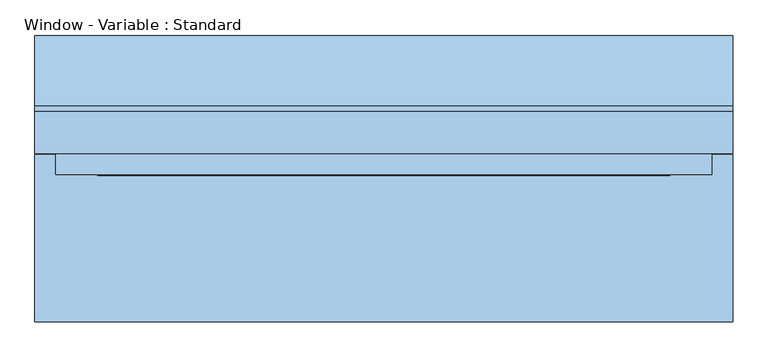
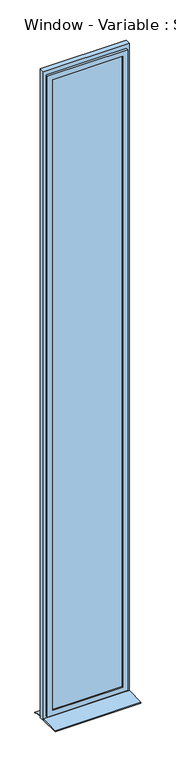
"""IFC4 building model written with IfcOpenShell, lengths in millimetres: window geometry, Window - Variable : Standard."""

import ifcopenshell
import ifcopenshell.guid

model = None  # the IFC model being written
_history = None  # IfcOwnerHistory: only IFC2X3 demands one
_inside = {}  # id of a spatial element -> (the spatial element, [elements in it])
_under = {}  # id of a project, library or spatial element -> (it, [spatial elements below it])
_declared = {}  # id of a project -> (the project, [libraries it declares])
_typed = {}  # id of a type object -> (the type object, [elements of that type])
_made_of = {}  # id of a material, layer set ... -> (it, [elements and type objects made of it])


def new_model(schema):
    """Start an empty IFC model of exactly this schema.

    Asked for "IFC4X3", IfcOpenShell would pick the latest addendum, in which some entities
    have other attributes; the version numbers below select the first issue.
    IFC2X3 requires an IfcOwnerHistory on every rooted entity: one is made here for all.
    """
    global model, _history
    if schema == "IFC4X3":
        model = ifcopenshell.file(schema_version=(4, 3, 0, 0))
    else:
        model = ifcopenshell.file(schema=schema)
    _inside.clear()
    _under.clear()
    _declared.clear()
    _typed.clear()
    _made_of.clear()
    _history = None
    if model.schema == "IFC2X3":
        org = make("IfcOrganization", Name="unknown")
        user = make(
            "IfcPersonAndOrganization",
            ThePerson=make("IfcPerson", FamilyName="unknown"),
            TheOrganization=org,
        )
        app = make(
            "IfcApplication",
            ApplicationDeveloper=org,
            Version="unknown",
            ApplicationFullName="unknown",
            ApplicationIdentifier="unknown",
        )
        _history = make(
            "IfcOwnerHistory",
            OwningUser=user,
            OwningApplication=app,
            ChangeAction="ADDED",
            CreationDate=0,
        )
    return model


def make(cls, **values):
    """One entity of the class cls with the attributes given. An attribute that is None is left unset."""
    return model.create_entity(
        cls, **{name: value for name, value in values.items() if value is not None}
    )


def rooted(cls, **values):
    """An entity with a GlobalId (a new one), such as an element, a storey or a relation."""
    return make(cls, GlobalId=ifcopenshell.guid.new(), OwnerHistory=_history, **values)


def si_unit(unit_type, name, prefix=None):
    """IfcSIUnit, for example si_unit("LENGTHUNIT", "METRE", prefix="MILLI")."""
    return make("IfcSIUnit", UnitType=unit_type, Prefix=prefix, Name=name)


def assignment(units):
    """IfcUnitAssignment: the units of a project."""
    return None if units is None else make("IfcUnitAssignment", Units=units)


def point(xyz):
    """IfcCartesianPoint."""
    return None if xyz is None else make("IfcCartesianPoint", Coordinates=xyz)


def direction(xyz):
    """IfcDirection."""
    return None if xyz is None else make("IfcDirection", DirectionRatios=xyz)


def frame(location, z_axis=None, x_axis=None):
    """IfcAxis2Placement3D, a coordinate frame: its origin and axes. An axis left out is left unset."""
    return make(
        "IfcAxis2Placement3D",
        Location=point(location),
        Axis=direction(z_axis),
        RefDirection=direction(x_axis),
    )


def origin():
    """The frame at (0, 0, 0) with its axes left unset."""
    return frame((0.0, 0.0, 0.0))


def place(relative_to, where):
    """IfcLocalPlacement: puts the frame where relative to a parent placement (None: the world)."""
    return make(
        "IfcLocalPlacement", PlacementRelTo=relative_to, RelativePlacement=where
    )


def context(
    kind, dimensions, precision=None, world=None, true_north=None, identifier=None
):
    """IfcGeometricRepresentationContext, for example the 3D "Model" context."""
    return make(
        "IfcGeometricRepresentationContext",
        ContextIdentifier=identifier,
        ContextType=kind,
        CoordinateSpaceDimension=dimensions,
        Precision=precision,
        WorldCoordinateSystem=world,
        TrueNorth=true_north,
    )


def project(units=None, contexts=None):
    """IfcProject with its units and contexts."""
    return rooted(
        "IfcProject",
        Name="project",
        RepresentationContexts=contexts,
        UnitsInContext=assignment(units),
    )


def spatial(cls, under=None, at=None, **own):
    """A site, building, storey or space (cls), placed at a placement, below another one or the project."""
    s = rooted(cls, ObjectPlacement=at, **own)
    if under is not None:
        _under.setdefault(under.id(), (under, []))[1].append(s)
    return s


def polyline(points):
    """IfcPolyline through the points."""
    return make("IfcPolyline", Points=[point(p) for p in points])


def outline(outer, holes=None, kind="AREA"):
    """IfcArbitraryClosedProfileDef: a profile drawn as a closed curve; with holes, ...WithVoids."""
    if holes is None:
        return make("IfcArbitraryClosedProfileDef", ProfileType=kind, OuterCurve=outer)
    return make(
        "IfcArbitraryProfileDefWithVoids",
        ProfileType=kind,
        OuterCurve=outer,
        InnerCurves=holes,
    )


def extrude(swept, where, along, depth):
    """IfcExtrudedAreaSolid: the profile swept, set in the frame where, extruded along a direction by depth."""
    return make(
        "IfcExtrudedAreaSolid",
        SweptArea=swept,
        Position=where,
        ExtrudedDirection=direction(along),
        Depth=depth,
    )


def faces_of(points, faces, orient=None, outer=None):
    """IfcFace entities. A face is a list of loops; a loop is a list of indices into points, from 0.

    orient and outer hold one flag for each loop. By default every Orientation is true, the
    first loop of a face is its IfcFaceOuterBound and the others are IfcFaceBound.
    """
    made = []
    for i, loops in enumerate(faces):
        bounds = []
        for j, loop in enumerate(loops):
            is_outer = j == 0 if outer is None else outer[i][j]
            bounds.append(
                make(
                    "IfcFaceOuterBound" if is_outer else "IfcFaceBound",
                    Bound=make("IfcPolyLoop", Polygon=[points[k] for k in loop]),
                    Orientation=True if orient is None else orient[i][j],
                )
            )
        made.append(make("IfcFace", Bounds=bounds))
    return made


def faceted_brep(points, faces, orient=None, outer=None, voids=None):
    """IfcFacetedBrep: a solid bounded by flat faces; with voids (closed shells), ...WithVoids."""
    shared = [point(p) for p in points]
    hull = make("IfcClosedShell", CfsFaces=faces_of(shared, faces, orient, outer))
    if voids is None:
        return make("IfcFacetedBrep", Outer=hull)
    return make(
        "IfcFacetedBrepWithVoids",
        Outer=hull,
        Voids=[
            make(cls, CfsFaces=faces_of(shared, fs, o, b)) for cls, fs, o, b in voids
        ],
    )


def shape(context_of_items, identifier, shape_type, items):
    """IfcShapeRepresentation: the items that make up one representation, for example the "Body"."""
    return make(
        "IfcShapeRepresentation",
        ContextOfItems=context_of_items,
        RepresentationIdentifier=identifier,
        RepresentationType=shape_type,
        Items=items,
    )


def source(mapping_origin, context_of_items, identifier, shape_type, items):
    """IfcRepresentationMap: a shape defined once, which mapped items show again and again."""
    return make(
        "IfcRepresentationMap",
        MappingOrigin=mapping_origin,
        MappedRepresentation=shape(context_of_items, identifier, shape_type, items),
    )


def transform(
    local_origin,
    x_axis=None,
    y_axis=None,
    z_axis=None,
    scale=None,
    scale2=None,
    scale3=None,
    uniform=True,
):
    """IfcCartesianTransformationOperator3D, or its non-uniform kind. x_axis, y_axis, z_axis: its Axis1, 2, 3."""
    if uniform:
        return make(
            "IfcCartesianTransformationOperator3D",
            Axis1=direction(x_axis),
            Axis2=direction(y_axis),
            LocalOrigin=point(local_origin),
            Scale=scale,
            Axis3=direction(z_axis),
        )
    return make(
        "IfcCartesianTransformationOperator3DnonUniform",
        Axis1=direction(x_axis),
        Axis2=direction(y_axis),
        LocalOrigin=point(local_origin),
        Scale=scale,
        Axis3=direction(z_axis),
        Scale2=scale2,
        Scale3=scale3,
    )


def mapped(mapping_source, mapping_target):
    """IfcMappedItem: shows the shape of a source again, moved by a transform."""
    return make(
        "IfcMappedItem", MappingSource=mapping_source, MappingTarget=mapping_target
    )


def made_of(thing, what):
    """Note that an element or type object is made of a material, layer set ...; save() writes the relation."""
    if what is not None:
        _made_of.setdefault(what.id(), (what, []))[1].append(thing)
    return thing


def element(
    cls,
    number,
    at=None,
    inside=None,
    cuts=None,
    type_object=None,
    material=None,
    context=None,
    identifier="Body",
    shape_type=None,
    held_by="IfcProductDefinitionShape",
    body=None,
    shapes=None,
    **own,
):
    """One element of the class cls, such as IfcWall. Its Tag is "e" and its number.

    at: its placement. inside: the storey or other place that contains it. cuts: it is an
    opening in that element (IfcRelVoidsElement). A single representation is given by context,
    identifier, shape_type and body (its items); several are given by shapes. held_by: the class
    of the entity that holds the representations. save() writes the other relations.
    """
    e = rooted(cls, Tag="e%d" % number, ObjectPlacement=at, **own)
    if body is not None:
        shapes = [shape(context, identifier, shape_type, body)]
    if shapes is not None:
        e.Representation = make(held_by, Representations=shapes)
    if inside is not None:
        _inside.setdefault(inside.id(), (inside, []))[1].append(e)
    if cuts is not None:
        rooted(
            "IfcRelVoidsElement", RelatingBuildingElement=cuts, RelatedOpeningElement=e
        )
    if type_object is not None:
        _typed.setdefault(type_object.id(), (type_object, []))[1].append(e)
    return made_of(e, material)


def aggregate(whole, parts):
    """IfcRelAggregates: a whole, such as a stair, and the parts it consists of."""
    return rooted("IfcRelAggregates", RelatingObject=whole, RelatedObjects=parts)


def save(model, path):
    """Write the relations noted so far, then the file.

    IfcRelAggregates (storeys below a building ...), IfcRelContainedInSpatialStructure (elements
    in a storey), IfcRelDefinesByType, IfcRelAssociatesMaterial and IfcRelDeclares: one each for
    every whole, place, type object, material and project.
    """
    for whole, parts in _under.values():
        aggregate(whole, parts)
    for where, things in _inside.values():
        rooted(
            "IfcRelContainedInSpatialStructure",
            RelatedElements=things,
            RelatingStructure=where,
        )
    for kind, things in _typed.values():
        rooted("IfcRelDefinesByType", RelatedObjects=things, RelatingType=kind)
    for what, things in _made_of.values():
        rooted("IfcRelAssociatesMaterial", RelatedObjects=things, RelatingMaterial=what)
    for by, libraries in _declared.values():
        rooted("IfcRelDeclares", RelatingContext=by, RelatedDefinitions=libraries)
    model.write(path)


def window_variable_standard_5cf830ff(model_context):
    return source(origin(), model_context, "Body", "SolidModel", [
        extrude(outline(polyline([(9000.0, 500.0), (9000.0, -500.0), (1000.0, -500.0), (1000.0, 500.0), (9000.0, 500.0)]), holes=[polyline([(8920.0, 440.0), (1080.0, 440.0), (1080.0, -440.0), (8920.0, -440.0), (8920.0, 440.0)])]), frame((0.0, 35.0, 0.0), z_axis=(0.0, 1.0, 0.0), x_axis=(0.0, 0.0, 1.0)), (0.0, 0.0, 1.0), 60.0),
        faceted_brep([(470.0, 35.0, 8950.0), (470.0, 5.0, 8950.0), (470.0, 5.0, 1050.0), (470.0, 35.0, 1050.0), (-470.0, 5.0, 8950.0), (-470.0, 5.0, 1050.0), (410.0, 5.0, 1110.0), (-410.0, 5.0, 1110.0), (-410.0, 5.0, 8890.0), (410.0, 5.0, 8890.0), (-470.0, 35.0, 1050.0), (-470.0, 35.0, 8950.0), (440.0, 35.0, 8920.0), (-440.0, 35.0, 8920.0), (-440.0, 35.0, 1080.0), (440.0, 35.0, 1080.0), (440.0, 65.0, 8920.0), (440.0, 65.0, 1080.0), (-440.0, 65.0, 1080.0), (-440.0, 65.0, 8920.0), (410.0, 65.0, 8890.0), (-410.0, 65.0, 8890.0), (-410.0, 65.0, 1110.0), (410.0, 65.0, 1110.0)], [[[0, 1, 2, 3]], [[1, 4, 5, 2], [6, 7, 8, 9]], [[3, 2, 5, 10]], [[3, 10, 11, 0], [12, 13, 14, 15]], [[16, 12, 15, 17]], [[17, 15, 14, 18]], [[17, 18, 19, 16], [20, 21, 22, 23]], [[9, 20, 23, 6]], [[6, 23, 22, 7]], [[10, 5, 4, 11]], [[18, 14, 13, 19]], [[7, 22, 21, 8]], [[11, 4, 1, 0]], [[19, 13, 12, 16]], [[8, 21, 20, 9]]]),
        extrude(outline(polyline([(-500.0, -205.0), (-500.0, 35.0), (500.0, 35.0), (500.0, -205.0), (-500.0, -205.0)])), frame((0.0, 0.0, 1005.0), z_axis=(0.0, 0.0, 1.0), x_axis=(1.0, 0.0, 0.0)), (0.0, 0.0, 1.0), 15.0),
        extrude(outline(polyline([(105.0221543, 1020.0), (205.0, 1000.0), (205.0, 990.0), (203.0, 990.0), (203.0, 998.3604634), (104.8240723, 1018.0), (95.0, 1018.0), (95.0, 1020.0), (105.0221543, 1020.0)])), frame((-500.0, 0.0, 0.0), z_axis=(1.0, 0.0, 0.0), x_axis=(0.0, 1.0, 0.0)), (0.0, 0.0, 1.0), 1000.0),
        extrude(outline(polyline([(410.0, 20.0), (-410.0, 20.0), (-410.0, 50.0), (410.0, 50.0), (410.0, 20.0)])), frame((0.0, 0.0, 1110.0), z_axis=(0.0, 0.0, 1.0), x_axis=(1.0, 0.0, 0.0)), (0.0, 0.0, 1.0), 7780.0),
    ])


if __name__ == "__main__":
    model = new_model("IFC4")
    model_context = context("Model", 3, world=origin())
    ifc_project = project(units=[si_unit("LENGTHUNIT", "METRE", prefix="MILLI")], contexts=[model_context])
    site = spatial("IfcSite", under=ifc_project)
    building = spatial("IfcBuilding", under=site)
    placement = place(None, origin())
    window_variable_standard_shape = window_variable_standard_5cf830ff(model_context)
    element("IfcWindow", 1, ObjectType="Window - Variable : Standard", at=placement, inside=building, context=model_context, shape_type="MappedRepresentation", body=[
        mapped(window_variable_standard_shape, transform((0.0, 0.0, 0.0), x_axis=(1.0, 0.0, 0.0), y_axis=(0.0, 1.0, 0.0), z_axis=(0.0, 0.0, 1.0))),
    ])
    save(model, "model.ifc")

# Revit data of these elements
# Type "Window - Variable : Standard"
#   Type Mark = "19"
#   Operation = "SinglePanel"
#   Keynote = "16.05.01"
#   Analytic Construction = "<None>"
#   Rough Width [instance default] = 1.010 m
#   Rough Height [instance default] = 1.010 m
#   Frame Depth = 0.060 m
#   Frame Height Bottom = 0.080 m
#   Frame Height Top = 0.080 m
#   Frame Width = 0.060 m
#   Height [instance default] = 1.010 m
#   Window Inset = 0.060 m
#   Window Width = 0.060 m
#   Instalation Depth [instance default] = 0.080 m
#   Width [instance default] = 1.010 m
#   Folding Wing [instance default] = no
#   Oppening Direction Vertical [instance default] = yes
#   Oppening Direction Visibility [instance default] = no
#   Casement [instance default] = yes
#   Frame [instance default] = none
#   Glas [instance default] = none
#   Window [instance default] = none
#   Windowsill Inside [instance default] = none
#   Windowsill Outside [instance default] = none
#   Wall Closure = (empty or 0)
#   Assembly Code = ""
# Element 1 (IfcWindow, "Window - Variable : Standard")
#   Rough Width = 1.000 m
#   Rough Height = 8.000 m
#   Height = 8.000 m
#   Width = 1.000 m
#   Materials on its faces: "Plastic - White", "Metal _ Aluminium", "Wood - Birch", "Glass"
# Materials
#   "Plastic - White": class "Kunststoff", colour RGB 249 249 249, transparency 0
#   "Metal _ Aluminium": class "Metall", colour RGB 247 247 247, transparency 0
#   "Wood - Birch": class "Holz", colour RGB 213 164 103, transparency 0
#   "Glass": class "Glass", colour RGB 0 128 192, transparency 0.9
